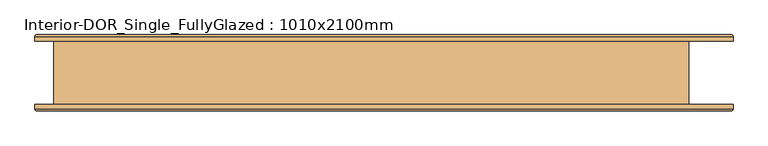
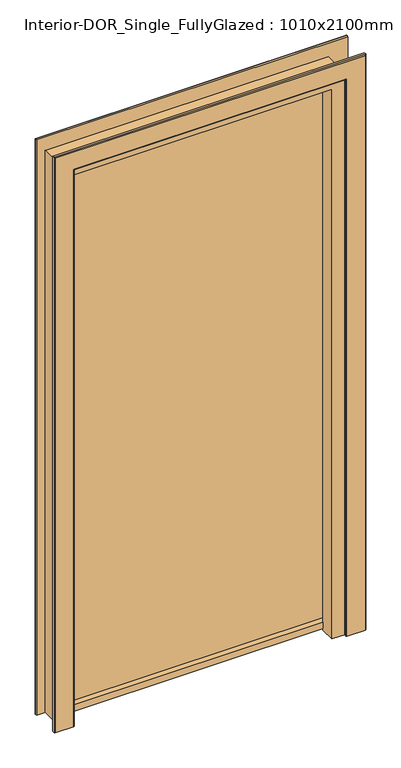
"""IFC4 building model written with IfcOpenShell, lengths in millimetres: door geometry, Interior-DOR_Single_FullyGlazed : 1010x2100mm."""

from ifc_helpers import new_model, si_unit, frame, origin, place, context, project, spatial, polyline, circle_curve, ellipse_curve, outline, extrude, faceted_brep, source, transform, mapped, element, save
from ifc_brep_helpers import plane_surface, cylinder_surface, advanced_brep


def interior_dor_single_fullyglazed_1010x2100mm_4e97d53e(model_context):
    return source(origin(), model_context, "Body", "SolidModel", [
        advanced_brep(
        [(-460.0, 50.0, 0.0), (-530.0, 50.0, 0.0), (-530.0, 57.0, 0.0), (-527.0, 60.0, 0.0), (-463.0, 60.0, 0.0), (-460.0, 57.0, 0.0), (-460.0, 57.0, 2075.0), (-460.0, 50.0, 2075.0), (-463.0, 60.0, 2078.0), (-527.0, 60.0, 2142.0), (567.0, 60.0, 2142.0), (567.0, 60.0, 0.0), (503.0, 60.0, 0.0), (503.0, 60.0, 2078.0), (-530.0, 57.0, 2145.0), (-530.0, 50.0, 2145.0), (500.0, 50.0, 2075.0), (500.0, 50.0, 0.0), (570.0, 50.0, 0.0), (570.0, 50.0, 2145.0), (500.0, 57.0, 0.0), (500.0, 57.0, 2075.0), (570.0, 57.0, 0.0), (570.0, 57.0, 2145.0)],
        [
            (0, 1),
            (1, 2),
            (2, 3, circle_curve(frame((-527.0, 57.0, 0.0), z_axis=(0.0, 0.0, -1.0), x_axis=(-1.0, 0.0, 0.0)), 3.0)),
            (3, 4),
            (4, 5, circle_curve(frame((-463.0, 57.0, 0.0), z_axis=(0.0, 0.0, -1.0), x_axis=(-1.0, 0.0, 0.0)), 3.0)),
            (5, 0),
            (5, 6),
            (6, 7),
            (7, 0),
            (4, 8),
            (8, 6, ellipse_curve(frame((-463.0, 57.0, 2078.0), z_axis=(-0.7071067811865475, 0.0, -0.7071067811865475), x_axis=(0.7071067811865474, 0.0, -0.7071067811865476)), 4.2426407, 3.0)),
            (3, 9),
            (9, 10),
            (10, 11),
            (11, 12),
            (12, 13),
            (13, 8),
            (2, 14),
            (14, 9, ellipse_curve(frame((-527.0, 57.0, 2142.0), z_axis=(-0.7071067811865475, 0.0, -0.7071067811865475), x_axis=(0.7071067811865474, 0.0, -0.7071067811865476)), 4.2426407, 3.0)),
            (1, 15),
            (15, 14),
            (7, 16),
            (16, 17),
            (17, 18),
            (18, 19),
            (19, 15),
            (12, 20, circle_curve(frame((503.0, 57.0, 0.0), z_axis=(0.0, 0.0, 1.0), x_axis=(1.0, 0.0, 0.0)), 3.0)),
            (20, 21),
            (21, 13, ellipse_curve(frame((503.0, 57.0, 2078.0), z_axis=(0.7071067811865475, 0.0, -0.7071067811865475), x_axis=(0.7071067811865474, 0.0, 0.7071067811865476)), 4.2426407, 3.0)),
            (17, 20),
            (11, 22, circle_curve(frame((567.0, 57.0, 0.0), z_axis=(0.0, 0.0, -1.0), x_axis=(1.0, 0.0, 0.0)), 3.0)),
            (22, 18),
            (23, 22),
            (10, 23, ellipse_curve(frame((567.0, 57.0, 2142.0), z_axis=(0.7071067811865475, 0.0, -0.7071067811865475), x_axis=(0.7071067811865474, 0.0, 0.7071067811865476)), 4.2426407, 3.0)),
            (23, 19),
            (16, 21),
            (6, 21),
            (14, 23),
        ],
        [
            plane_surface(frame((-480.0, -50.0, 0.0), z_axis=(0.0, 0.0, -1.0), x_axis=(0.0, 1.0, 0.0))),
            plane_surface(frame((-460.0, 50.0, 0.0), z_axis=(1.0, 0.0, 0.0), x_axis=(0.0, 0.0, 1.0))),
            cylinder_surface(frame((-463.0, 57.0, 0.0), z_axis=(0.0, 0.0, -1.0), x_axis=(-1.0, 0.0, 0.0)), 3.0),
            plane_surface(frame((-463.0, 60.0, 0.0), z_axis=(0.0, 1.0, 0.0), x_axis=(0.0, 0.0, 1.0))),
            cylinder_surface(frame((-527.0, 57.0, 0.0), z_axis=(0.0, 0.0, -1.0), x_axis=(-1.0, 0.0, 0.0)), 3.0),
            plane_surface(frame((-530.0, 57.0, 0.0), z_axis=(-1.0, 0.0, 0.0), x_axis=(0.0, 0.0, 1.0))),
            plane_surface(frame((-530.0, 50.0, 0.0), z_axis=(0.0, -1.0, 0.0), x_axis=(0.0, 0.0, 1.0))),
            cylinder_surface(frame((503.0, 57.0, 2095.0), z_axis=(0.0, 0.0, 1.0), x_axis=(1.0, 0.0, 0.0)), 3.0),
            plane_surface(frame((520.0, -50.0, 0.0), z_axis=(0.0, 0.0, -1.0), x_axis=(0.0, 1.0, 0.0))),
            cylinder_surface(frame((567.0, 57.0, 2095.0), z_axis=(0.0, 0.0, 1.0), x_axis=(1.0, 0.0, 0.0)), 3.0),
            plane_surface(frame((570.0, 57.0, 2145.0), z_axis=(1.0, 0.0, 0.0), x_axis=(0.0, 0.0, -1.0))),
            plane_surface(frame((500.0, 50.0, 2075.0), z_axis=(-1.0, 0.0, 0.0), x_axis=(0.0, 0.0, -1.0))),
            plane_surface(frame((-460.0, 50.0, 2075.0), z_axis=(0.0, 0.0, -1.0), x_axis=(1.0, 0.0, 0.0))),
            cylinder_surface(frame((-480.0, 57.0, 2078.0), z_axis=(-1.0, 0.0, 0.0), x_axis=(0.0, 0.0, 1.0)), 3.0),
            cylinder_surface(frame((-480.0, 57.0, 2142.0), z_axis=(-1.0, 0.0, 0.0), x_axis=(0.0, 0.0, 1.0)), 3.0),
            plane_surface(frame((-530.0, 57.0, 2145.0), z_axis=(0.0, 0.0, 1.0), x_axis=(1.0, 0.0, 0.0))),
        ],
        [
            (0, [[1, 2, 3, 4, 5, 6]]),
            (1, [[7, 8, 9, -6]]),
            (2, [[10, 11, -7, -5]]),
            (3, [[12, 13, 14, 15, 16, 17, -10, -4]]),
            (4, [[18, 19, -12, -3]]),
            (5, [[20, 21, -18, -2]]),
            (6, [[-9, 22, 23, 24, 25, 26, -20, -1]]),
            (7, [[-16, 27, 28, 29]]),
            (8, [[30, -27, -15, 31, 32, -24]]),
            (9, [[33, -31, -14, 34]]),
            (10, [[-25, -32, -33, 35]]),
            (11, [[-28, -30, -23, 36]]),
            (12, [[37, -36, -22, -8]]),
            (13, [[-17, -29, -37, -11]]),
            (14, [[38, -34, -13, -19]]),
            (15, [[-26, -35, -38, -21]]),
        ],
    ),
        advanced_brep(
        [(-530.0, -50.0, 0.0), (-460.0, -50.0, 0.0), (-460.0, -57.0, 0.0), (-463.0, -60.0, 0.0), (-527.0, -60.0, 0.0), (-530.0, -57.0, 0.0), (-530.0, -57.0, 2145.0), (-530.0, -50.0, 2145.0), (-527.0, -60.0, 2142.0), (-463.0, -60.0, 2078.0), (503.0, -60.0, 2078.0), (503.0, -60.0, 0.0), (567.0, -60.0, 0.0), (567.0, -60.0, 2142.0), (-460.0, -57.0, 2075.0), (-460.0, -50.0, 2075.0), (570.0, -50.0, 2145.0), (570.0, -50.0, 0.0), (500.0, -50.0, 0.0), (500.0, -50.0, 2075.0), (570.0, -57.0, 0.0), (570.0, -57.0, 2145.0), (500.0, -57.0, 0.0), (500.0, -57.0, 2075.0)],
        [
            (0, 1),
            (1, 2),
            (2, 3, circle_curve(frame((-463.0, -57.0, 0.0), z_axis=(0.0, 0.0, -1.0), x_axis=(-1.0, 0.0, 0.0)), 3.0)),
            (3, 4),
            (4, 5, circle_curve(frame((-527.0, -57.0, 0.0), z_axis=(0.0, 0.0, -1.0), x_axis=(-1.0, 0.0, 0.0)), 3.0)),
            (5, 0),
            (5, 6),
            (6, 7),
            (7, 0),
            (4, 8),
            (8, 6, ellipse_curve(frame((-527.0, -57.0, 2142.0), z_axis=(-0.7071067811865475, 0.0, -0.7071067811865475), x_axis=(0.7071067811865474, 0.0, -0.7071067811865476)), 4.2426407, 3.0)),
            (3, 9),
            (9, 10),
            (10, 11),
            (11, 12),
            (12, 13),
            (13, 8),
            (2, 14),
            (14, 9, ellipse_curve(frame((-463.0, -57.0, 2078.0), z_axis=(-0.7071067811865475, 0.0, -0.7071067811865475), x_axis=(0.7071067811865474, 0.0, -0.7071067811865476)), 4.2426407, 3.0)),
            (1, 15),
            (15, 14),
            (7, 16),
            (16, 17),
            (17, 18),
            (18, 19),
            (19, 15),
            (12, 20, circle_curve(frame((567.0, -57.0, 0.0), z_axis=(0.0, 0.0, 1.0), x_axis=(1.0, 0.0, 0.0)), 3.0)),
            (20, 21),
            (21, 13, ellipse_curve(frame((567.0, -57.0, 2142.0), z_axis=(0.7071067811865475, 0.0, -0.7071067811865475), x_axis=(0.7071067811865474, 0.0, 0.7071067811865476)), 4.2426407, 3.0)),
            (17, 20),
            (11, 22, circle_curve(frame((503.0, -57.0, 0.0), z_axis=(0.0, 0.0, -1.0), x_axis=(1.0, 0.0, 0.0)), 3.0)),
            (22, 18),
            (23, 22),
            (10, 23, ellipse_curve(frame((503.0, -57.0, 2078.0), z_axis=(0.7071067811865475, 0.0, -0.7071067811865475), x_axis=(0.7071067811865474, 0.0, 0.7071067811865476)), 4.2426407, 3.0)),
            (23, 19),
            (16, 21),
            (6, 21),
            (14, 23),
        ],
        [
            plane_surface(frame((-480.0, -50.0, 0.0), z_axis=(0.0, 0.0, -1.0), x_axis=(0.0, 1.0, 0.0))),
            plane_surface(frame((-530.0, -50.0, 0.0), z_axis=(-1.0, 0.0, 0.0), x_axis=(0.0, 0.0, 1.0))),
            cylinder_surface(frame((-527.0, -57.0, 0.0), z_axis=(0.0, 0.0, -1.0), x_axis=(-1.0, 0.0, 0.0)), 3.0),
            plane_surface(frame((-527.0, -60.0, 0.0), z_axis=(0.0, -1.0, 0.0), x_axis=(0.0, 0.0, 1.0))),
            cylinder_surface(frame((-463.0, -57.0, 0.0), z_axis=(0.0, 0.0, -1.0), x_axis=(-1.0, 0.0, 0.0)), 3.0),
            plane_surface(frame((-460.0, -57.0, 0.0), z_axis=(1.0, 0.0, 0.0), x_axis=(0.0, 0.0, 1.0))),
            plane_surface(frame((-460.0, -50.0, 0.0), z_axis=(0.0, 1.0, 0.0), x_axis=(0.0, 0.0, 1.0))),
            cylinder_surface(frame((567.0, -57.0, 2095.0), z_axis=(0.0, 0.0, 1.0), x_axis=(1.0, 0.0, 0.0)), 3.0),
            plane_surface(frame((520.0, -50.0, 0.0), z_axis=(0.0, 0.0, -1.0), x_axis=(0.0, 1.0, 0.0))),
            cylinder_surface(frame((503.0, -57.0, 2095.0), z_axis=(0.0, 0.0, 1.0), x_axis=(1.0, 0.0, 0.0)), 3.0),
            plane_surface(frame((500.0, -57.0, 2075.0), z_axis=(-1.0, 0.0, 0.0), x_axis=(0.0, 0.0, -1.0))),
            plane_surface(frame((570.0, -50.0, 2145.0), z_axis=(1.0, 0.0, 0.0), x_axis=(0.0, 0.0, -1.0))),
            plane_surface(frame((-530.0, -50.0, 2145.0), z_axis=(0.0, 0.0, 1.0), x_axis=(1.0, 0.0, 0.0))),
            cylinder_surface(frame((-480.0, -57.0, 2142.0), z_axis=(-1.0, 0.0, 0.0), x_axis=(0.0, 0.0, 1.0)), 3.0),
            cylinder_surface(frame((-480.0, -57.0, 2078.0), z_axis=(-1.0, 0.0, 0.0), x_axis=(0.0, 0.0, 1.0)), 3.0),
            plane_surface(frame((-460.0, -57.0, 2075.0), z_axis=(0.0, 0.0, -1.0), x_axis=(1.0, 0.0, 0.0))),
        ],
        [
            (0, [[1, 2, 3, 4, 5, 6]]),
            (1, [[7, 8, 9, -6]]),
            (2, [[10, 11, -7, -5]]),
            (3, [[12, 13, 14, 15, 16, 17, -10, -4]]),
            (4, [[18, 19, -12, -3]]),
            (5, [[20, 21, -18, -2]]),
            (6, [[-9, 22, 23, 24, 25, 26, -20, -1]]),
            (7, [[-16, 27, 28, 29]]),
            (8, [[30, -27, -15, 31, 32, -24]]),
            (9, [[33, -31, -14, 34]]),
            (10, [[-25, -32, -33, 35]]),
            (11, [[-28, -30, -23, 36]]),
            (12, [[37, -36, -22, -8]]),
            (13, [[-17, -29, -37, -11]]),
            (14, [[38, -34, -13, -19]]),
            (15, [[-26, -35, -38, -21]]),
        ],
    ),
        extrude(outline(polyline([(470.0, 31.0), (470.0, 24.0), (-430.0, 24.0), (-430.0, 31.0), (470.0, 31.0)])), frame((0.0, 0.0, 30.0), z_axis=(0.0, 0.0, 1.0), x_axis=(1.0, 0.0, 0.0)), (0.0, 0.0, 1.0), 2015.0),
        extrude(outline(polyline([(5.0, -455.0), (5.0, 495.0), (2070.0, 495.0), (2070.0, -455.0), (5.0, -455.0)]), holes=[polyline([(2045.0, 470.0), (30.0, 470.0), (30.0, -430.0), (2045.0, -430.0), (2045.0, 470.0)])]), frame((0.0, 5.0, 0.0), z_axis=(0.0, 1.0, 0.0), x_axis=(0.0, 0.0, 1.0)), (0.0, 0.0, 1.0), 45.0),
        faceted_brep([(-500.0, -50.0, 0.0), (-500.0, 50.0, 0.0), (-475.0, 50.0, 0.0), (-475.0, 5.0, 0.0), (-455.0, 5.0, 0.0), (-455.0, -50.0, 0.0), (-455.0, -50.0, 2050.0), (455.0, -50.0, 2050.0), (455.0, -50.0, 0.0), (500.0, -50.0, 0.0), (500.0, -50.0, 2095.0), (-500.0, -50.0, 2095.0), (-455.0, 5.0, 2050.0), (-475.0, 5.0, 2070.0), (475.0, 5.0, 2070.0), (475.0, 5.0, 0.0), (455.0, 5.0, 0.0), (455.0, 5.0, 2050.0), (-475.0, 50.0, 2070.0), (-500.0, 50.0, 2095.0), (500.0, 50.0, 2095.0), (500.0, 50.0, 0.0), (475.0, 50.0, 0.0), (475.0, 50.0, 2070.0)], [[[0, 1, 2, 3, 4, 5]], [[5, 6, 7, 8, 9, 10, 11, 0]], [[4, 12, 6, 5]], [[3, 13, 14, 15, 16, 17, 12, 4]], [[2, 18, 13, 3]], [[1, 19, 20, 21, 22, 23, 18, 2]], [[0, 11, 19, 1]], [[10, 9, 21, 20]], [[9, 8, 16, 15, 22, 21]], [[17, 16, 8, 7]], [[23, 22, 15, 14]], [[12, 17, 7, 6]], [[18, 23, 14, 13]], [[11, 10, 20, 19]]]),
    ])


if __name__ == "__main__":
    model = new_model("IFC4")
    model_context = context("Model", 3, world=origin())
    ifc_project = project(units=[si_unit("LENGTHUNIT", "METRE", prefix="MILLI")], contexts=[model_context])
    site = spatial("IfcSite", under=ifc_project)
    building = spatial("IfcBuilding", under=site)
    placement = place(None, origin())
    interior_dor_single_fullyglazed_1010x2100mm_shape = interior_dor_single_fullyglazed_1010x2100mm_4e97d53e(model_context)
    element("IfcDoor", 1, ObjectType="Interior-DOR_Single_FullyGlazed : 1010x2100mm", at=placement, inside=building, context=model_context, shape_type="MappedRepresentation", body=[
        mapped(interior_dor_single_fullyglazed_1010x2100mm_shape, transform((0.0, 0.0, 0.0), x_axis=(1.0, 0.0, 0.0), y_axis=(0.0, 1.0, 0.0), z_axis=(0.0, 0.0, 1.0))),
    ])
    save(model, "model.ifc")

# Revit data of these elements
# Type "Interior-DOR_Single_FullyGlazed : 1010x2100mm"
#   Type IfcGUID = "2NKTNbJKP36hSTtB23u7pq"
#   Type Mark = "187"
#   Classification.Uniclass.EF.Number = "EF_25_30"
#   Classification.Uniclass.EF.Description = "Doors and windows"
#   WindLoadRating = "n/a"
#   WaterTightnessRating = "n/a"
#   WarrantyStartDate [instance default] = "1900-12-31T23:59:59"
#   WarrantyGuarantorParts = "n/a"
#   WarrantyGuarantorLabor = "n/a"
#   WarrantyDurationUnit = "year"
#   WarrantyDurationParts = "n/a"
#   WarrantyDurationLabor = "n/a"
#   WarrantyDescription = "n/a"
#   Version = "2"
#   Uniclass2015Version = "Systems v1.9"
#   Uniclass2015Title = "Doorset systems"
#   Uniclass2015Code = "Ss_25_30_20_25"
#   URL = "www.nationalbimlibrary.com"
#   TagNumber [instance default] = "n/a"
#   SustainabilityPerformance = "n/a"
#   Status = "UNSET"
#   Size = "1010 x 2100 mm"
#   Shape = "n/a"
#   SerialNumber [instance default] = "n/a"
#   SecurityRating = "n/a"
#   Revision = "n/a"
#   ReplacementCost = "n/a"
#   Reference = "n/a"
#   ProductInformation = "n/a"
#   Operation = "SINGLE_SWING_RIGHT"
#   OmniClassVersion = "Table 22 2012-05-16"
#   OmniClassTitle = "Doors and Frames"
#   OmniClassCode = "22-08 10 00"
#   Name = "DoorsetSystem_Interior-Single_FullyGlazed"
#   NBSReference = "25-50-20/120"
#   NBSDescription = "Doorset system"
#   NBSCertification = "www.nationalbimlibrary.com/cert/43bi5322"
#   ModelReference = "Interior Single Door Fully Glazed Leaf"
#   ModelNumber = "n/a"
#   Model = "Interior Single Door Fully Glazed Leaf"
#   MechanicalLoadRating = "n/a"
#   Material = "n/a"
#   ManufacturerURL = "n/a"
#   ManufacturerName = "n/a"
#   Manufacturer = "info@theNBS.com"
#   InstallationDate [instance default] = "1900-12-31T23:59:59"
#   IfcExportType = "DOOR"
#   IfcExportAs = "IfcDoorType"
#   HygrothermalRating = "n/a"
#   Grade = "n/a"
#   GlassColor = "n/a"
#   FireRating = "n/a"
#   Fire Rating = "n/a"
#   Finish = "n/a"
#   FillGas = "n/a"
#   Features = "n/a"
#   ExpectedLife = "n/a"
#   DurationUnit = "n/a"
#   DurabilityRating = "n/a"
#   DoorNumber [instance default] = "n/a"
#   Description = "Generic single interior door with fully glazed leaf"
#   Construction Type = "USERDEFINED"
#   Constituents = "n/a"
#   ComponentNumber [instance default] = "n/a"
#   Color = "n/a"
#   CodePerformance = "n/a"
#   Category = "Ss_25_30_20_25:Doorset systems"
#   BarCode [instance default] = "n/a"
#   BIMObjectName = "NBS_DoorsetSystem_Interior-Single_FullyGlazed"
#   Author = "NBS"
#   AssetType = "Fixed"
#   AssetIdentifier [instance default] = "n/a"
#   AcousticRating = "n/a"
#   AccessibilityPerformance = "n/a"
#   WallThickness [instance default] = 0.15 m
#   VisibleLightTransmittance = 0
#   VisibileLightReflectance = 0
#   ThresholdHeight = 0.015 m
#   ThermalTransmittanceWinter = 0
#   ThermalTransmittanceSummer = 0
#   ThermalTransmittance = 0
#   StructuralToleranceJamb = 0.005 m
#   StructuralToleranceHead = 0.005 m
#   StructuralOpeningWidth = 1.01 m
#   StructuralOpeningHeight = 2.1 m
#   StructuralOpeningCutBeyondFaceInternalMinimum [instance default] = 0.005 m
#   StructuralOpeningCutBeyondFaceInternal [instance default] = 0.005 m
#   StructuralOpeningCutBeyondFaceExternal [instance default] = 0.005 m
#   StopProjection = 0.02 m
#   StopDepth = 0.04 m
#   SolarTransmittance = 0
#   SolarReflectance = 0
#   SolarHeatGainTransmittance = 0
#   SolarAbsorption = 0
#   ShadingCoefficient = 0
#   RebateDepth = 0.045 m
#   PanelWidth = 0.95 m
#   PanelHeight = 2.07 m
#   PanelDepth = 0.045 m
#   OpeningTolerance = 0 m
#   NominalWidth = 1.01 m
#   NominalLength = 0 m
#   NominalHeight = 2.1 m
#   PanelUndercut = 0.005 m
#   LayerWrapExternal [instance default] = 0.005 m
#   Infiltration = 0
#   GlazingPanelThickness = 0.007 m
#   GlazingCavityThicknessOuter = 0 m
#   GlazingCavityThicknessIntermediate = 0 m
#   GlazingCavityThicknessInner = 0 m
#   GlazingAreaFraction = 0
#   GlassThickness3 = 0.002 m
#   GlassThickness2 = 0.002 m
#   GlassThickness1 = 0.002 m
#   FrameThickness = 0.025 m
#   FrameSetback [instance default] = 0 m
#   FrameDepth [instance default] = 0.15 m
#   Height = 2.1 m
#   Width = 1.01 m
#   FinishThicknessInternal [instance default] = 0 m
#   FinishThicknessExternal [instance default] = 0 m
#   ClearOpeningWidth = 0.91 m
#   ClearOpeningHeight = 2.05 m
#   ArchitraveWidth = 0.07 m
#   ArchitraveThickness = 0.01 m
#   ArchitraveSetbackFromFrameFace = 0.005 m
#   SmokeStop = no
#   SingleRebate = yes
#   SelfClosing = no
#   PlantedStop = no
#   IsWired = no
#   IsTempered = no
#   IsLaminated = no
#   IsExternal = no
#   IsCoated = no
#   HasDrive = no
#   HandicapAccessible = no
#   GlazingUnitTriple = yes
#   GlazingUnitDouble = no
#   GlassLayers = 3
#   Wall Closure = 4
#   FireExit = no
#   PanelMaterial = NBS_Concept
#   GlazingPanelMaterial = NBS_Glass_Single
#   GlazingBeadMaterial = NBS_Concept
#   FrameSectionMaterial = NBS_Concept
#   Function = (empty or 0)
#   Cost = 0
# Element 1 (IfcDoor, "Interior-DOR_Single_FullyGlazed : 1010x2100mm")
#   WallThickness = 0.1 m
#   FrameDepth = 0.1 m
#   Materials on its faces: "NBS_Concept", "NBS_Glass_Single"
# Materials
#   "NBS_Concept": class "Generic", colour RGB 255 255 255, transparency 0, Description = "To be specified", Cost = 0
#   "NBS_Glass_Single": class "Glass", colour RGB 94 140 251, transparency 0.6, Cost = 0
